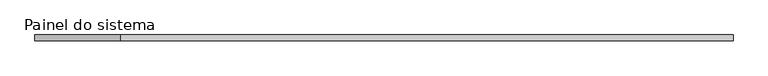
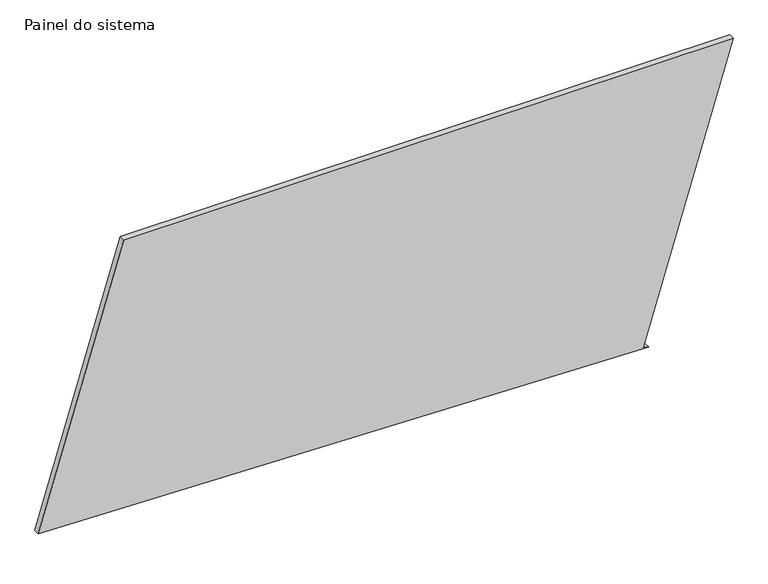
"""IFC4 building model written with IfcOpenShell, lengths in millimetres: plate geometry, Painel do sistema : Envidraçado."""

from ifc_helpers import new_model, si_unit, frame, origin, place, context, project, spatial, polyline, outline, extrude, source, transform, mapped, element, save


def painel_do_sistema_b63d67f1(model_context):
    return source(origin(), model_context, "Body", "SweptSolid", [
        extrude(outline(polyline([(0.0, 1149.2587263), (7.2712141, 1125.3394987), (1298.9323194, 1517.9919958), (1298.9323194, -1144.7496726), (71.1224994, -1517.9919958), (0.0, 1149.2587263)])), frame((0.0, 24.5, 0.0), z_axis=(0.0, 1.0, 0.0), x_axis=(0.0, 0.0, 1.0)), (0.0, 0.0, 1.0), 25.0),
    ])


if __name__ == "__main__":
    model = new_model("IFC4")
    model_context = context("Model", 3, world=origin())
    ifc_project = project(units=[si_unit("LENGTHUNIT", "METRE", prefix="MILLI")], contexts=[model_context])
    site = spatial("IfcSite", under=ifc_project)
    building = spatial("IfcBuilding", under=site)
    placement = place(None, origin())
    painel_do_sistema_shape = painel_do_sistema_b63d67f1(model_context)
    element("IfcPlate", 1, ObjectType="Painel do sistema : Envidraçado", at=placement, inside=building, context=model_context, shape_type="MappedRepresentation", body=[
        mapped(painel_do_sistema_shape, transform((0.0, 0.0, 0.0), x_axis=(1.0, 0.0, 0.0), y_axis=(0.0, 1.0, 0.0), z_axis=(0.0, 0.0, 1.0))),
    ])
    save(model, "model.ifc")

# Revit data of these elements
# Type "Painel do sistema : Envidraçado"
#   Construction Type Id = "GSP4R"
#   Analytic Construction = "Vidraça única Pilkington 1/8 pol"
#   Visual Light Transmittance = 0.9
#   Solar Heat Gain Coefficient = 0.86
#   Heat Transfer Coefficient (U) = 6.7069 W/(m²·K)
# Element 1 (IfcPlate, "Painel do sistema : Envidraçado")
#   Materials on its faces: "Vidro"
# Materials
#   "Vidro": class "Vidro", colour RGB 0 128 192, transparency 0.9, Description = "Vidro de sílica", Cost = 0
